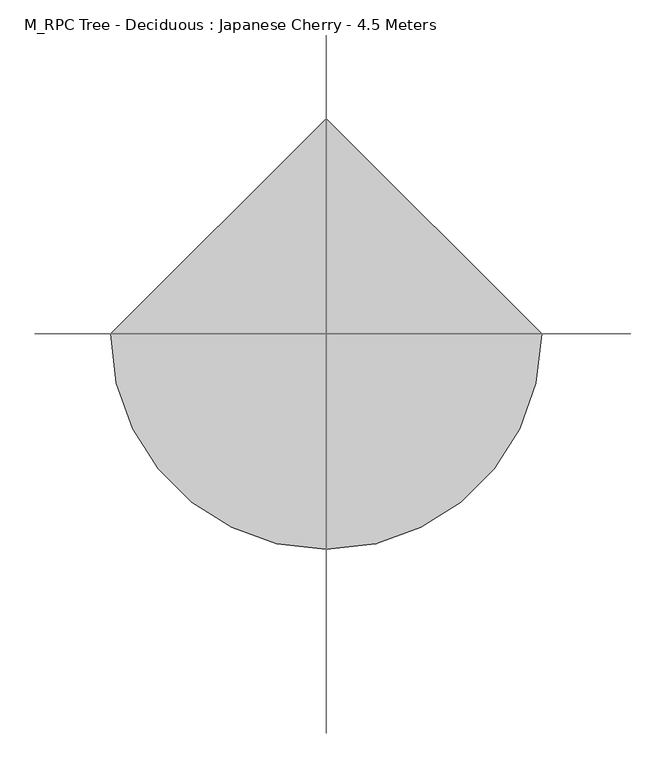
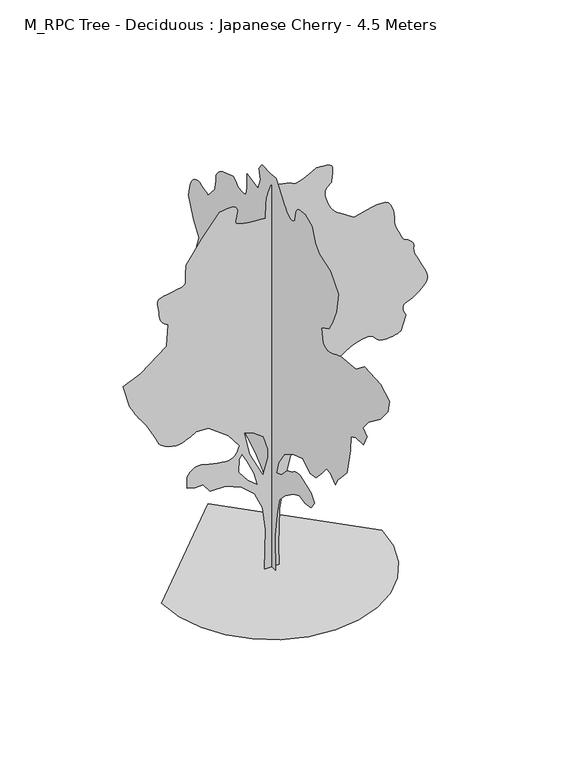
"""IFC4 building model written with IfcOpenShell, lengths in millimetres: geographic element geometry, M_RPC Tree - Deciduous : Japanese Cherry - 4.5 Meters."""

from ifc_helpers import new_model, si_unit, origin, place, context, project, spatial, triangles, source, transform, mapped, element, save


def m_rpc_tree_deciduous_japanese_cherry_4_5_meters_7aaeb41d(model_context):
    return source(origin(), model_context, "Body", "Tessellation", [
        triangles([(-0.0027587, 74.5725603, 0.00586), (-0.0027587, -72.0943095, 0.00586), (-0.0027587, -58.7610481, 393.3378007), (-0.0027587, -98.7608322, 653.338028), (-0.0027587, -145.4276149, 853.3381748), (-0.0027587, -252.0952047, 966.670792), (-0.0027587, -412.0928332, 1080.00588), (-0.0027587, -518.7604139, 1126.6709095), (-0.0027587, -625.428031, 1106.6708948), (-0.0027587, -738.7605755, 1126.6709095), (-0.0027587, -798.7606195, 1213.3385118), (-0.0027587, -738.7605755, 1293.3384979), (-0.0027587, -525.4279212, 1366.6710857), (-0.0027587, -506.885412, 1365.1761189), (-0.0027587, -488.5178922, 1363.2711479), (-0.0027587, -470.5003873, 1360.5486397), (-0.0027587, -453.0078504, 1356.6035316), (-0.0027587, -436.2153434, 1351.0261105), (-0.0027587, -420.2953485, 1343.4060814), (-0.0027587, -405.4278331, 1333.3385273), (-0.0027587, -390.5578105, 1322.4935497), (-0.0027587, -374.6402864, 1312.6960373), (-0.0027587, -357.8477795, 1303.7760876), (-0.0027587, -340.3552789, 1295.553479), (-0.0027587, -322.337774, 1287.8585999), (-0.0027587, -303.9702541, 1280.5110832), (-0.0027587, -285.4277268, 1273.3385559), (-0.0027587, -185.427399, 1166.6709389), (-0.0027587, -85.4275708, 1126.6709095), (-0.0027587, -125.4276002, 1266.671085), (-0.0027587, -238.7606988, 1433.3386734), (-0.0027587, -398.7603258, 1533.3386742), (-0.0027587, -585.4279653, 1593.3387909), (-0.0027587, -718.7605608, 1506.6712612), (-0.0027587, -825.4281778, 1520.0062031), (-0.0027587, -938.7607224, 1640.0038204), (-0.0027587, -1025.4283247, 1746.6714375), (-0.0027587, -1105.4259127, 1740.0039665), (-0.0027587, -1192.0934423, 1660.0063786), (-0.0027587, -1245.4260155, 1753.3389084), (-0.0027587, -1305.4259869, 1820.0040253), (-0.0027587, -1412.0936039, 1933.3391132), (-0.0027587, -1478.7587208, 2233.3392609), (-0.0027587, -1485.4261917, 2393.3393784), (-0.0027587, -1578.7613377, 2433.336937), (-0.0027587, -1725.426368, 2446.6718788), (-0.0027587, -1785.4264847, 2573.3269386), (-0.0027587, -1712.0938969, 2633.3270554), (-0.0027587, -1812.0938976, 2753.3272888), (-0.0027587, -2038.759132, 2926.6774635), (-0.0027587, -2185.4267784, 3100.0026398), (-0.0027587, -2212.0917206, 3240.0025246), (-0.0027587, -2045.4266029, 3333.3276421), (-0.0027587, -1738.758839, 3346.6776993), (-0.0027587, -1585.4263378, 3226.6774658), (-0.0027587, -1292.0935158, 3193.3274666), (-0.0027587, -1252.2485641, 3177.7025482), (-0.0027587, -1213.3385118, 3162.6025978), (-0.0027587, -1176.2909185, 3148.5525833), (-0.0027587, -1142.0459158, 3136.0774727), (-0.0027587, -1111.5309179, 3125.7025246), (-0.0027587, -1085.6808969, 3117.9524162), (-0.0027587, -1065.4258833, 3113.3274078), (-0.0027587, -1047.2933418, 3113.0774231), (-0.0027587, -1028.108321, 3117.0274727), (-0.0027587, -1009.2758223, 3123.6526497), (-0.0027587, -992.1908186, 3131.4524643), (-0.0027587, -978.255768, 3138.9025909), (-0.0027587, -968.8682596, 3144.4775414), (-0.0027587, -965.4258099, 3146.6774071), (-0.0027587, -932.0932514, 3306.6778152), (-0.0027587, -1072.0933542, 3380.0027), (-0.0027587, -1138.7609419, 3486.6778748), (-0.0027587, -1212.093457, 3660.003051), (-0.0027587, -1252.0934864, 3880.0029945), (-0.0027587, -1098.7609125, 4053.3281708), (-0.0027587, -898.760693, 4126.6783447), (-0.0027587, -818.7606342, 4200.0035202), (-0.0027587, -758.7605902, 4360.0036377), (-0.0027587, -618.7604874, 4413.3285805), (-0.0027587, -595.9604982, 4413.2285866), (-0.0027587, -573.5129585, 4412.5536278), (-0.0027587, -551.7629416, 4410.70345), (-0.0027587, -531.0629333, 4407.1286682), (-0.0027587, -511.7629123, 4401.17845), (-0.0027587, -494.2128934, 4392.3534073), (-0.0027587, -478.7603846, 4380.0035797), (-0.0027587, -466.2228868, 4364.5536507), (-0.0027587, -456.8353784, 4347.0035591), (-0.0027587, -450.0728551, 4327.7035744), (-0.0027587, -445.4078419, 4307.0033844), (-0.0027587, -442.3178415, 4285.2535492), (-0.0027587, -440.2753427, 4262.803466), (-0.0027587, -438.7603552, 4240.0034042), (-0.0027587, -427.2553525, 4227.3033073), (-0.0027587, -415.2803204, 4215.6034401), (-0.0027587, -402.3753304, 4205.9034508), (-0.0027587, -388.070317, 4199.1532814), (-0.0027587, -371.9003011, 4196.3784508), (-0.0027587, -353.3952896, 4198.553318), (-0.0027587, -332.0927745, 4206.6784035), (-0.0027587, -310.9852693, 4218.4782646), (-0.0027587, -293.0277353, 4231.0033722), (-0.0027587, -277.6927156, 4244.1034447), (-0.0027587, -264.4552061, 4257.6784882), (-0.0027587, -252.7927094, 4271.5785118), (-0.0027587, -242.1814384, 4285.7285202), (-0.0027587, -232.0939364, 4300.003521), (-0.0027587, -138.7608616, 4426.6786377), (-0.0027587, -78.7608175, 4500.0035225), (-0.0027587, 21.2393172, 4493.3286392), (-0.0027587, 181.2391554, 4500.0035225), (-0.0027587, 241.2389451, 4420.0034637), (-0.0027587, 214.5724224, 4306.6784042), (-0.0027587, 261.2402133, 4180.0032875), (-0.0027587, 467.9053785, 4220.0034622), (-0.0027587, 467.9053785, 4073.3284035), (-0.0027587, 469.4403866, 4050.6283356), (-0.0027587, 471.6178699, 4028.7032204), (-0.0027587, 475.0778695, 4008.4282951), (-0.0027587, 480.4628969, 3990.6282188), (-0.0027587, 488.4103769, 3976.0532364), (-0.0027587, 499.5679081, 3965.5782944), (-0.0027587, 514.5729152, 3960.0030533), (-0.0027587, 531.7154371, 3957.9281799), (-0.0027587, 548.8579591, 3957.2532211), (-0.0027587, 566.0004447, 3957.7281921), (-0.0027587, 583.1429667, 3959.1531052), (-0.0027587, 600.2854886, 3961.2782661), (-0.0027587, 617.4304813, 3963.853109), (-0.0027587, 634.5730396, 3966.6782272), (-0.0027587, 650.2955538, 3982.2281502), (-0.0027587, 666.0780207, 3996.928125), (-0.0027587, 681.9780676, 4009.8782066), (-0.0027587, 698.0505604, 4020.2031578), (-0.0027587, 714.3580679, 4027.0283226), (-0.0027587, 730.9580721, 4029.4781731), (-0.0027587, 747.9055841, 4026.678344), (-0.0027587, 927.9057163, 3966.6782272), (-0.0027587, 953.4457998, 3949.4781143), (-0.0027587, 977.9358021, 3931.9283134), (-0.0027587, 1000.3257872, 3913.6782646), (-0.0027587, 1019.5682899, 3894.3782799), (-0.0027587, 1034.6108311, 3873.6780899), (-0.0027587, 1044.4058727, 3851.2280067), (-0.0027587, 1047.9058771, 3826.6780518), (-0.0027587, 1048.6833733, 3801.5281334), (-0.0027587, 1050.8608566, 3777.4531494), (-0.0027587, 1054.2033852, 3754.253112), (-0.0027587, 1058.4783422, 3731.7530319), (-0.0027587, 1063.4533293, 3709.7529213), (-0.0027587, 1068.895875, 3688.1280785), (-0.0027587, 1074.570892, 3666.6779343), (-0.0027587, 1201.238451, 3526.6777588), (-0.0027587, 1239.7609543, 3543.5528915), (-0.0027587, 1277.9935043, 3558.9278252), (-0.0027587, 1315.641061, 3571.2779434), (-0.0027587, 1352.4135258, 3579.077758), (-0.0027587, 1388.0210907, 3580.8029434), (-0.0027587, 1422.1711864, 3574.9530098), (-0.0027587, 1454.5712437, 3560.0027596), (-0.0027587, 1482.6961258, 3536.9027161), (-0.0027587, 1504.8736965, 3508.1777252), (-0.0027587, 1522.093721, 3474.8027275), (-0.0027587, 1535.3487259, 3437.7026665), (-0.0027587, 1545.6312378, 3397.8027763), (-0.0027587, 1553.9313126, 3356.02771), (-0.0027587, 1561.2387154, 3313.3277), (-0.0027587, 1474.5711857, 3086.677581), (-0.0027587, 1367.9060394, 2940.0022316), (-0.0027587, 1454.5712437, 2700.0020554), (-0.0027587, 1374.5710396, 2573.3269386), (-0.0027587, 1341.9185268, 2561.8270592), (-0.0027587, 1310.4910847, 2549.851918), (-0.0027587, 1281.5110222, 2536.952124), (-0.0027587, 1256.2035553, 2522.6521248), (-0.0027587, 1235.7959347, 2506.4769493), (-0.0027587, 1221.5110508, 2487.9745903), (-0.0027587, 1214.5709948, 2466.6721115), (-0.0027587, 1212.2984591, 2444.0095413), (-0.0027587, 1211.0734612, 2421.694479), (-0.0027587, 1210.7234825, 2399.6744568), (-0.0027587, 1211.0734612, 2377.8869785), (-0.0027587, 1211.9484804, 2356.2718735), (-0.0027587, 1213.1734783, 2334.7768192), (-0.0027587, 1214.5709948, 2313.3368488), (-0.0027587, 1187.9059799, 2206.6718479), (-0.0027587, 1001.2383041, 2226.6717899), (-0.0027587, 985.728277, 2195.3792233), (-0.0027587, 971.4433205, 2164.9017231), (-0.0027587, 959.6057436, 2136.0592976), (-0.0027587, 951.4432331, 2109.6642517), (-0.0027587, 948.1782434, 2086.536739), (-0.0027587, 951.0357725, 2067.486739), (-0.0027587, 961.2382748, 2053.3392014), (-0.0027587, 977.7782536, 2041.5992203), (-0.0027587, 998.0507807, 2029.6266953), (-0.0027587, 1020.8883402, 2018.0041489), (-0.0027587, 1045.1258142, 2007.3141037), (-0.0027587, 1069.5958323, 1998.1390823), (-0.0027587, 1093.133349, 1991.0640781), (-0.0027587, 1114.5709213, 1986.6716137), (-0.0027587, 1133.9884134, 1982.8416149), (-0.0027587, 1152.3558969, 1977.2640484), (-0.0027587, 1169.8484339, 1970.229158), (-0.0027587, 1186.6409409, 1962.0266064), (-0.0027587, 1202.9109507, 1952.9491081), (-0.0027587, 1218.828511, 1943.2890873), (-0.0027587, 1234.5710094, 1933.3391132), (-0.0027587, 1387.9061268, 2013.339172), (-0.0027587, 1431.9861397, 2024.5916828), (-0.0027587, 1474.8436981, 2034.7965832), (-0.0027587, 1515.2512608, 2042.9016117), (-0.0027587, 1551.9862278, 2047.8566872), (-0.0027587, 1583.8238194, 2048.6141991), (-0.0027587, 1609.5388195, 2044.1266823), (-0.0027587, 1627.9038322, 2033.339114), (-0.0027587, 1640.0538174, 2017.6916679), (-0.0027587, 1648.351276, 1999.5965515), (-0.0027587, 1653.4438431, 1979.4615887), (-0.0027587, 1655.9713051, 1957.6915512), (-0.0027587, 1656.5738846, 1934.6990593), (-0.0027587, 1655.8938389, 1910.8890301), (-0.0027587, 1654.5713905, 1886.6714676), (-0.0027587, 1631.6563648, 1862.5890713), (-0.0027587, 1608.3913605, 1839.7339256), (-0.0027587, 1584.4262535, 1819.3239796), (-0.0027587, 1559.4112106, 1802.5889545), (-0.0027587, 1532.9962532, 1790.7539211), (-0.0027587, 1504.833728, 1785.0390083), (-0.0027587, 1474.5711857, 1786.6714668), (-0.0027587, 1442.5211071, 1793.7065025), (-0.0027587, 1410.0036152, 1802.1439236), (-0.0027587, 1378.1860806, 1810.1114605), (-0.0027587, 1348.2360191, 1815.7489071), (-0.0027587, 1321.3160053, 1817.1864647), (-0.0027587, 1298.5960258, 1812.5614563), (-0.0027587, 1281.2385098, 1800.0039379), (-0.0027587, 1268.1185257, 1783.8339947), (-0.0027587, 1257.0985588, 1769.4114738), (-0.0027587, 1247.8260143, 1756.448893), (-0.0027587, 1239.9560005, 1744.6513573), (-0.0027587, 1233.1334518, 1733.7264427), (-0.0027587, 1227.0110058, 1723.3863762), (-0.0027587, 1221.2385384, 1713.338879), (-0.0027587, 1243.9585178, 1710.3264175), (-0.0027587, 1265.8635761, 1706.3813095), (-0.0027587, 1286.1360306, 1700.5688736), (-0.0027587, 1303.9584892, 1691.958934), (-0.0027587, 1318.5160309, 1679.6163734), (-0.0027587, 1328.993589, 1662.608836), (-0.0027587, 1334.5710102, 1640.0038204), (-0.0027587, 1336.8460167, 1613.5138676), (-0.0027587, 1338.0710873, 1585.6212387), (-0.0027587, 1338.4210659, 1556.56371), (-0.0027587, 1338.0710873, 1526.5736801), (-0.0027587, 1337.1961407, 1495.8836929), (-0.0027587, 1335.9710701, 1464.7286179), (-0.0027587, 1334.5710102, 1433.3386734), (-0.0027587, 1300.3260075, 1407.8185741), (-0.0027587, 1266.3110779, 1383.4636654), (-0.0027587, 1232.7635616, 1361.4436432), (-0.0027587, 1199.9160027, 1342.9210819), (-0.0027587, 1168.0034157, 1329.0636429), (-0.0027587, 1137.2534031, 1321.0360806), (-0.0027587, 1107.9059212, 1320.0060562), (-0.0027587, 1078.5558958, 1323.638538), (-0.0027587, 1047.808354, 1328.6735504), (-0.0027587, 1015.8932962, 1334.873608), (-0.0027587, 983.0458099, 1342.0060215), (-0.0027587, 949.4982937, 1349.8411537), (-0.0027587, 915.4857622, 1358.1386124), (-0.0027587, 881.238216, 1366.6710857), (-0.0027587, 681.2380692, 1320.0060562), (-0.0027587, 447.9053638, 1200.0059681), (-0.0027587, 314.5727683, 1126.6709095), (-0.0027587, 161.2391225, 1000.0058212), (-0.0027587, 67.905807, 806.6731453), (-0.0027587, 41.2392842, 533.3379398), (-0.0027587, 67.905807, 260.0052052), (78.9470616, 0.0002511, 0.0), (-81.0528197, 0.0002511, 0.0), (-67.7195538, 0.0002197, 453.3328669), (-101.05258, 0.0001988, 713.3330578), (-187.7194103, 0.0001884, 899.9982628), (-327.7202579, 0.0001884, 1026.6658218), (-501.0529192, 0.0001779, 1099.9984097), (-667.7180368, 0.0001779, 1099.9984097), (-747.720639, 0.0001779, 1199.9984831), (-834.3856979, 0.0001779, 1199.9984831), (-921.0532276, 0.0001779, 1219.9984978), (-921.0532276, 0.0001674, 1346.6660568), (-903.7932346, 0.0001674, 1369.3085701), (-885.8332117, 0.0001674, 1390.6686035), (-866.4756723, 0.000157, 1409.4636772), (-845.0181885, 0.000157, 1424.411166), (-820.7606575, 0.000157, 1434.2261192), (-793.0056656, 0.000157, 1437.6286732), (-761.0531101, 0.000157, 1433.3335865), (-723.1130568, 0.000157, 1423.7311203), (-679.5755253, 0.000157, 1412.8461742), (-633.0054754, 0.0001674, 1401.8461189), (-585.970483, 0.0001674, 1391.8936741), (-541.032928, 0.0001674, 1384.1586811), (-500.7604225, 0.0001674, 1379.803569), (-467.71789, 0.0001674, 1379.9986153), (-441.4803563, 0.0001674, 1385.9661289), (-419.4403499, 0.0001674, 1397.5311207), (-400.8978407, 0.000157, 1413.7610893), (-385.1527988, 0.000157, 1433.7212082), (-371.5103176, 0.000157, 1456.4811562), (-359.2652802, 0.000157, 1481.1062519), (-347.7202726, 0.000157, 1506.6661743), (-467.71789, 0.0001465, 1666.6662918), (-687.7180515, 0.000136, 1826.6664093), (-821.0531542, 0.000136, 1833.3314095), (-842.5681927, 0.000136, 1820.5039948), (-864.6081991, 0.000136, 1807.851424), (-887.7006849, 0.000136, 1795.5489773), (-912.3632057, 0.000136, 1783.7688824), (-939.1282871, 0.000136, 1772.6913609), (-968.5158102, 0.000136, 1762.4864605), (-1001.0532864, 0.0001465, 1753.3313507), (-1038.4858126, 0.0001465, 1750.1639568), (-1080.1183731, 0.0001465, 1756.5589153), (-1122.8009422, 0.000136, 1770.6488983), (-1163.385965, 0.000136, 1790.5713741), (-1198.7209448, 0.000136, 1814.4590149), (-1225.6584721, 0.000136, 1840.4465275), (-1241.0509918, 0.000136, 1866.6664387), (-1254.4834568, 0.000136, 1899.3565945), (-1275.8434902, 0.0001256, 1942.8940533), (-1302.4510231, 0.0001256, 1992.6141289), (-1331.6261318, 0.0001256, 2043.8466122), (-1360.6836605, 0.0001256, 2091.9317585), (-1386.9410694, 0.0001151, 2132.204155), (-1407.7185802, 0.0001151, 2159.9992607), (-1425.2510857, 0.0001151, 2182.1367176), (-1443.4812229, 0.0001151, 2208.1242302), (-1462.2962082, 0.0001151, 2237.3167797), (-1481.576136, 0.0001151, 2269.0742889), (-1501.2061878, 0.0001046, 2302.7592968), (-1521.0712543, 0.0001046, 2337.7244591), (-1541.0512848, 0.0001046, 2373.3318787), (-1614.3863434, 9.42e-05, 2626.6771706), (-1421.0511967, 8.37e-05, 2706.6772293), (-1141.0533892, 7.32e-05, 2926.6774635), (-1127.7183746, 5.23e-05, 3166.6526413), (-1147.5834412, 5.23e-05, 3181.0776329), (-1166.6309704, 5.23e-05, 3196.1775833), (-1184.0459684, 5.23e-05, 3212.677739), (-1199.0109707, 5.23e-05, 3231.2774757), (-1210.7109833, 5.23e-05, 3252.677623), (-1218.3310123, 5.23e-05, 3277.5775566), (-1221.0535206, 5.23e-05, 3306.6525261), (-1223.4635479, 4.19e-05, 3339.402562), (-1228.9034775, 4.19e-05, 3373.552803), (-1234.6960018, 4.19e-05, 3407.2527809), (-1238.155965, 4.19e-05, 3438.6029022), (-1236.6009727, 4.19e-05, 3465.7526985), (-1227.3484852, 4.19e-05, 3486.8278656), (-1207.7185061, 4.19e-05, 3500.0029335), (-1173.335939, 4.19e-05, 3508.2777191), (-1126.1258846, 3.14e-05, 3516.4528015), (-1072.8508661, 3.14e-05, 3525.1778503), (-1020.2758049, 3.14e-05, 3535.2278183), (-975.1632969, 3.14e-05, 3547.2279579), (-944.2782635, 3.14e-05, 3561.9279327), (-934.3857714, 3.14e-05, 3580.0029922), (-936.4657316, 3.14e-05, 3601.7528275), (-937.1457773, 3.14e-05, 3626.6530518), (-936.6582344, 3.14e-05, 3654.1778252), (-935.2407337, 3.14e-05, 3683.7780533), (-933.1232758, 2.09e-05, 3714.9778931), (-930.5382591, 2.09e-05, 3747.2279594), (-927.7182278, 2.09e-05, 3780.0029938), (-761.0531101, 1.05e-05, 4020.00317), (-567.7204705, -1.05e-05, 4260.0033463), (-526.5729095, -1.05e-05, 4266.8535095), (-487.1179049, -1.05e-05, 4272.0284843), (-451.042854, -1.05e-05, 4273.8283745), (-420.0428567, -1.05e-05, 4270.5285759), (-395.80531, -1.05e-05, 4260.4783173), (-380.0228067, -1.05e-05, 4241.9782837), (-374.3852875, 0.0, 4213.3282883), (-377.165314, 0.0, 4181.0535141), (-383.5603088, 0.0, 4152.6032158), (-390.6553336, 0.0, 4127.8032761), (-395.5328339, 0.0, 4106.3534225), (-395.2803057, 0.0, 4088.0533768), (-386.9803036, 0.0, 4072.6781525), (-367.7202873, 0.0, 4060.0033447), (-338.5077899, 0.0, 4049.7283905), (-302.995241, 0.0, 4041.5783066), (-262.2377179, 1.05e-05, 4035.1531174), (-217.282177, 1.05e-05, 4030.1531319), (-169.1771373, 1.05e-05, 4026.1783745), (-118.9730978, 1.05e-05, 4022.9032837), (-67.7195538, 1.05e-05, 4020.00317), (-61.0525507, 0.0, 4200.0035202), (-59.4975493, -1.05e-05, 4225.5284157), (-55.1437952, -1.05e-05, 4250.678334), (-48.4577889, -1.05e-05, 4275.5535599), (-39.9057809, -1.05e-05, 4300.2035088), (-29.954274, -1.05e-05, 4324.6784683), (-19.070066, -1.05e-05, 4349.0284355), (-7.719256, -1.05e-05, 4373.3284058), (37.7812808, -1.05e-05, 4364.72864), (81.9990646, -1.05e-05, 4356.0285896), (123.6511007, -1.05e-05, 4347.103553), (161.4548797, -1.05e-05, 4337.8035393), (194.127413, -1.05e-05, 4328.053553), (220.3859302, -1.05e-05, 4317.7036034), (238.9474425, -1.05e-05, 4306.6534058), (263.1077047, -1.05e-05, 4303.4286026), (302.4252358, -1.05e-05, 4313.503569), (350.0252918, -1.05e-05, 4332.2035904), (399.0253169, -1.05e-05, 4354.8786598), (442.5428641, -1.05e-05, 4376.8284828), (473.6978665, -2.09e-05, 4393.4286324), (485.6129096, -2.09e-05, 4400.0035217), (495.2154121, -2.09e-05, 4400.2035095), (519.9779268, -2.09e-05, 4399.9285263), (553.8354532, -2.09e-05, 4397.9036499), (590.7254617, -2.09e-05, 4392.8536674), (624.5830244, -1.05e-05, 4383.4786583), (649.3455391, -1.05e-05, 4368.5034096), (658.9480053, -1.05e-05, 4346.6535805), (658.5580582, -1.05e-05, 4321.3283821), (657.4705519, -1.05e-05, 4296.7034317), (655.7980522, -1.05e-05, 4272.6784447), (653.6605373, -1.05e-05, 4249.1034302), (651.1730438, -1.05e-05, 4225.8783943), (648.4505356, 0.0, 4202.8783447), (645.6129908, 0.0, 4180.0032875), (628.6255102, 0.0, 4167.0034996), (612.5730017, 0.0, 4153.2784653), (598.3829885, 0.0, 4138.0032349), (586.992986, 0.0, 4120.4784325), (579.3354592, 0.0, 4099.9282333), (576.342982, 0.0, 4075.5782661), (578.9479829, 0.0, 4046.6532875), (586.2154899, 1.05e-05, 4014.6032089), (596.2829713, 1.05e-05, 3981.953167), (608.6854846, 1.05e-05, 3949.7530975), (622.9504932, 1.05e-05, 3919.0782257), (638.6155254, 1.05e-05, 3890.9781967), (655.2155296, 1.05e-05, 3866.4782387), (672.280549, 2.09e-05, 3846.6529953), (692.3380457, 2.09e-05, 3828.553228), (717.6455853, 2.09e-05, 3808.6779877), (747.3231342, 2.09e-05, 3787.3531265), (780.5031584, 2.09e-05, 3764.8780449), (816.3031534, 2.09e-05, 3741.5030182), (853.853187, 2.09e-05, 3717.5780251), (892.2807106, 2.09e-05, 3693.3280518), (959.140801, 2.09e-05, 3711.6280975), (1024.3108057, 2.09e-05, 3728.2279564), (1086.098386, 2.09e-05, 3741.4280228), (1142.8159269, 2.09e-05, 3749.5781067), (1192.7659304, 2.09e-05, 3750.9530228), (1234.2634701, 2.09e-05, 3743.8781639), (1265.6135914, 2.09e-05, 3726.6530525), (1288.19855, 2.09e-05, 3698.6530174), (1305.0685959, 3.14e-05, 3662.6028923), (1317.0411209, 3.14e-05, 3621.8780525), (1324.9335171, 3.14e-05, 3579.8779999), (1329.5585255, 3.14e-05, 3539.9778191), (1331.7360088, 4.19e-05, 3505.5528854), (1332.2810337, 4.19e-05, 3480.0027008), (1337.451067, 4.19e-05, 3452.7529106), (1350.7835381, 4.19e-05, 3414.6526199), (1369.0136753, 4.19e-05, 3371.2026558), (1388.8785965, 5.23e-05, 3327.8526855), (1407.1112045, 5.23e-05, 3290.1026642), (1420.4436756, 5.23e-05, 3263.4275482), (1425.6137089, 5.23e-05, 3253.3275833), (1432.59119, 5.23e-05, 3250.5527527), (1450.4136486, 5.23e-05, 3242.5276611), (1474.4187241, 5.23e-05, 3229.7275703), (1499.938678, 5.23e-05, 3212.6024529), (1522.3086788, 5.23e-05, 3191.6275703), (1536.8662205, 5.23e-05, 3167.2776031), (1538.9461807, 6.28e-05, 3140.0025238), (1536.3412525, 6.28e-05, 3112.1024826), (1539.3362732, 6.28e-05, 3085.0273911), (1546.9938, 6.28e-05, 3057.9525902), (1558.3838024, 6.28e-05, 3030.0775475), (1572.5713085, 6.28e-05, 3000.5523148), (1588.6262878, 7.32e-05, 2968.5775223), (1605.6137684, 7.32e-05, 2933.3273483), (1625.0112762, 7.32e-05, 2895.102356), (1646.5088013, 7.32e-05, 2855.2271736), (1666.4888317, 7.32e-05, 2814.5523308), (1681.3363266, 8.37e-05, 2773.8771973), (1687.4413319, 8.37e-05, 2734.0023056), (1681.1813942, 8.37e-05, 2695.7773132), (1658.9462688, 8.37e-05, 2660.0021713), (1628.9963528, 9.42e-05, 2628.8270393), (1601.3762363, 9.42e-05, 2603.2521469), (1575.1563251, 9.42e-05, 2582.3269707), (1549.4036819, 9.42e-05, 2565.1521469), (1523.1837708, 9.42e-05, 2550.7771523), (1495.5662704, 9.42e-05, 2538.2520447), (1465.6137383, 9.42e-05, 2526.6771698), (1440.211219, 9.42e-05, 2513.3021141), (1425.6512066, 9.42e-05, 2496.4220398), (1420.1311947, 9.42e-05, 2476.6369102), (1421.8435902, 0.0001046, 2454.5170395), (1428.976149, 0.0001046, 2430.6494556), (1439.7236034, 0.0001046, 2405.616972), (1452.2811218, 0.0001046, 2379.9993496), (1398.9461506, 0.0001151, 2213.3317612), (1380.1910454, 0.0001151, 2204.8392563), (1360.3261242, 0.0001151, 2196.8118393), (1338.2460766, 0.0001151, 2189.7167782), (1312.8435574, 0.0001151, 2184.021777), (1283.0086052, 0.0001151, 2180.194249), (1247.6334389, 0.0001151, 2178.6968113), (1205.6134747, 0.0001151, 2179.9992027), (1167.8684675, 0.0001151, 2188.6467854), (1142.0184465, 0.0001151, 2205.9268353), (1121.9983749, 0.0001151, 2227.4043034), (1101.7459047, 0.0001151, 2248.6467567), (1075.1958538, 0.0001151, 2265.2268494), (1036.2833307, 0.0001151, 2272.7093868), (978.9457695, 0.0001151, 2266.6642616), (912.6507608, 0.0001151, 2247.8318356), (851.8331795, 0.0001151, 2221.3017689), (797.8981722, 0.0001151, 2189.1717533), (752.2406393, 0.0001151, 2153.5467476), (716.2655823, 0.0001151, 2116.5192112), (691.365576, 0.0001256, 2080.1942482), (678.94802, 0.0001256, 2046.6666435), (678.6755802, 0.0001256, 2016.7915775), (688.1980368, 0.0001256, 1989.7166313), (705.8855473, 0.0001256, 1964.9741009), (730.1031097, 0.0001256, 1942.0990437), (759.2181204, 0.000136, 1920.6215755), (791.6006641, 0.000136, 1900.0764633), (825.6131956, 0.000136, 1879.9990551), (845.4582052, 0.000136, 1867.0540604), (864.3707136, 0.000136, 1853.5839523), (881.4156761, 0.000136, 1839.0665245), (895.6632076, 0.000136, 1822.9739021), (906.1782635, 0.000136, 1804.7814079), (912.0282698, 0.000136, 1783.9639286), (912.2807253, 0.000136, 1759.998967), (909.6182425, 0.0001465, 1730.7863605), (907.3057383, 0.0001465, 1695.2763187), (905.28326, 0.0001465, 1654.5187775), (903.4957237, 0.0001465, 1609.5613472), (901.880706, 0.000157, 1561.4562893), (900.3857391, 0.000157, 1511.253685), (898.9457108, 0.000157, 1459.998674), (864.6231691, 0.000157, 1434.5760979), (830.0656855, 0.000157, 1410.9037056), (795.0406431, 0.0001674, 1390.7286289), (759.3156435, 0.0001674, 1375.8010517), (722.6606134, 0.0001674, 1367.8711578), (684.835524, 0.0001674, 1368.686079), (645.6129908, 0.0001674, 1379.9986153), (606.1979911, 0.0001674, 1395.0036587), (567.8304565, 0.0001674, 1406.1611172), (530.3354342, 0.000157, 1414.1112133), (493.5429125, 0.000157, 1419.4935883), (457.2753588, 0.000157, 1422.9536968), (421.3578564, 0.000157, 1425.1311802), (385.6127998, 0.000157, 1426.6661156), (272.280219, 0.0001674, 1353.3335278), (198.9474132, 0.0001779, 1186.6659393), (125.6138534, 0.0001884, 906.6657337), (85.6140693, 0.0002093, 633.332999), (72.2805581, 0.0002302, 233.3331958), (-94.386072, 8.37e-05, 1079.998395), (-41.0527812, 7.32e-05, 1266.6659981), (-41.0527812, 6.28e-05, 1359.9985279), (-87.7190734, 5.23e-05, 1519.9987907), (-207.7189163, 5.23e-05, 1606.6663204), (-301.052736, 5.23e-05, 1639.9988789), (-241.0526919, 6.28e-05, 1373.3336151), (-154.3856164, 6.28e-05, 993.3333361), (-194.385664, 6.28e-05, 1139.998439), (-267.7202139, 5.23e-05, 1299.9985565), (-321.0527507, 4.19e-05, 1399.9987026), (-354.3852728, 4.19e-05, 1353.3335278), (-361.0527801, 5.23e-05, 1206.665954), (-261.0527066, 6.28e-05, 1079.998395), (-1193.8159389, 0.0, 0.0045206), (-1162.2559467, -273.5427146, 0.0045206), (-1072.3708809, -524.7504189, 0.0045206), (-931.360738, -746.420573, 0.0045206), (-746.420573, -931.360738, 0.0045206), (-524.7504189, -1072.3708809, 0.0045206), (-273.5427146, -1162.2559467, 0.0045206), (5.22e-05, -1193.8159389, 0.0045206), (273.5427146, -1162.2559467, 0.0045206), (524.7504189, -1072.3708809, 0.0045206), (746.420573, -931.360738, 0.0045206), (931.360738, -746.420573, 0.0045206), (1072.3708809, -524.7504189, 0.0045206), (1162.2559467, -273.5427146, 0.0045206), (1193.8159389, 0.0001046, 0.0045206), (-0.0001566, 1193.8159389, 0.0045206)], [[38, 39, 40], [115, 116, 117], [1, 2, 3], [280, 1, 3], [279, 280, 3], [279, 3, 4], [278, 279, 4], [278, 4, 5], [186, 187, 188], [277, 278, 5], [46, 47, 48], [45, 46, 48], [277, 5, 6], [185, 186, 188], [10, 11, 12], [9, 10, 12], [9, 12, 13], [8, 9, 13], [8, 13, 14], [8, 14, 15], [8, 15, 16], [8, 16, 17], [8, 17, 18], [8, 18, 19], [8, 19, 20], [8, 20, 21], [7, 8, 21], [7, 21, 22], [7, 22, 23], [7, 23, 24], [7, 24, 25], [7, 25, 26], [6, 7, 26], [6, 26, 27], [6, 27, 28], [277, 6, 28], [277, 28, 29], [51, 52, 53], [50, 51, 53], [50, 53, 54], [50, 54, 55], [49, 50, 55], [49, 55, 56], [48, 49, 56], [48, 56, 57], [45, 48, 57], [44, 45, 57], [44, 57, 58], [44, 58, 59], [44, 59, 60], [44, 60, 61], [44, 61, 62], [44, 62, 63], [276, 277, 29], [276, 29, 30], [184, 185, 188], [183, 184, 188], [44, 63, 64], [115, 117, 118], [111, 112, 113], [111, 113, 114], [182, 183, 188], [109, 110, 111], [109, 111, 114], [108, 109, 114], [108, 114, 115], [107, 108, 115], [106, 107, 115], [105, 106, 115], [104, 105, 115], [115, 118, 119], [170, 171, 172], [170, 172, 173], [170, 173, 174], [170, 174, 175], [74, 75, 76], [74, 76, 77], [73, 74, 77], [72, 73, 77], [71, 72, 77], [258, 259, 260], [181, 182, 188], [78, 79, 80], [170, 175, 176], [103, 104, 115], [78, 80, 81], [44, 64, 65], [275, 276, 30], [275, 30, 31], [274, 275, 31], [78, 81, 82], [78, 82, 83], [78, 83, 84], [78, 84, 85], [78, 85, 86], [78, 86, 87], [78, 87, 88], [78, 88, 89], [78, 89, 90], [78, 90, 91], [78, 91, 92], [78, 92, 93], [78, 93, 94], [78, 94, 95], [78, 95, 96], [71, 77, 78], [71, 78, 96], [71, 96, 97], [71, 97, 98], [71, 98, 99], [71, 99, 100], [115, 119, 120], [180, 181, 188], [38, 40, 41], [223, 224, 225], [33, 34, 35], [33, 35, 36], [33, 36, 37], [102, 103, 115], [179, 180, 188], [44, 65, 66], [170, 176, 177], [71, 100, 101], [43, 44, 66], [42, 43, 66], [41, 42, 66], [38, 41, 66], [37, 38, 66], [33, 37, 66], [33, 66, 67], [33, 67, 68], [33, 68, 69], [33, 69, 70], [32, 33, 70], [31, 32, 70], [274, 31, 70], [273, 274, 70], [273, 70, 71], [273, 71, 101], [273, 101, 102], [273, 102, 115], [273, 115, 120], [273, 120, 121], [273, 121, 122], [273, 122, 123], [273, 123, 124], [273, 124, 125], [273, 125, 126], [273, 126, 127], [273, 127, 128], [273, 128, 129], [273, 129, 130], [273, 130, 131], [272, 273, 131], [271, 272, 131], [270, 271, 131], [269, 270, 131], [268, 269, 131], [268, 131, 132], [268, 132, 133], [268, 133, 134], [167, 168, 169], [257, 258, 260], [257, 260, 261], [256, 257, 261], [256, 261, 262], [255, 256, 262], [255, 262, 263], [254, 255, 263], [254, 263, 264], [254, 264, 265], [254, 265, 266], [254, 266, 267], [254, 267, 268], [253, 254, 268], [252, 253, 268], [251, 252, 268], [250, 251, 268], [249, 250, 268], [248, 249, 268], [247, 248, 268], [246, 247, 268], [245, 246, 268], [166, 167, 169], [165, 166, 169], [164, 165, 169], [163, 164, 169], [162, 163, 169], [161, 162, 169], [160, 161, 169], [159, 160, 169], [158, 159, 169], [157, 158, 169], [156, 157, 169], [155, 156, 169], [154, 155, 169], [154, 169, 170], [154, 170, 177], [153, 154, 177], [153, 177, 178], [153, 178, 179], [153, 179, 188], [222, 223, 225], [222, 225, 226], [221, 222, 226], [220, 221, 226], [219, 220, 226], [218, 219, 226], [217, 218, 226], [216, 217, 226], [215, 216, 226], [214, 215, 226], [213, 214, 226], [212, 213, 226], [212, 226, 227], [212, 227, 228], [212, 228, 229], [212, 229, 230], [212, 230, 231], [211, 212, 231], [211, 231, 232], [211, 232, 233], [210, 211, 233], [209, 210, 233], [209, 233, 234], [209, 234, 235], [209, 235, 236], [209, 236, 237], [209, 237, 238], [209, 238, 239], [209, 239, 240], [208, 209, 240], [208, 240, 241], [207, 208, 241], [206, 207, 241], [206, 241, 242], [205, 206, 242], [204, 205, 242], [204, 242, 243], [203, 204, 243], [202, 203, 243], [202, 243, 244], [201, 202, 244], [201, 244, 245], [201, 245, 268], [200, 201, 268], [199, 200, 268], [198, 199, 268], [197, 198, 268], [196, 197, 268], [195, 196, 268], [194, 195, 268], [153, 188, 189], [153, 189, 190], [152, 153, 190], [152, 190, 191], [151, 152, 191], [136, 137, 138], [135, 136, 138], [135, 138, 139], [134, 135, 139], [134, 139, 140], [134, 140, 141], [134, 141, 142], [134, 142, 143], [134, 143, 144], [134, 144, 145], [134, 145, 146], [134, 146, 147], [134, 147, 148], [134, 148, 149], [134, 149, 150], [134, 150, 151], [134, 151, 191], [134, 191, 192], [134, 192, 193], [268, 134, 193], [194, 268, 193], [583, 580, 581], [574, 281, 575], [580, 583, 584], [573, 574, 575], [583, 581, 575], [580, 584, 585], [572, 573, 575], [582, 583, 575], [582, 575, 281], [571, 572, 575], [571, 575, 576], [281, 282, 283], [570, 571, 576], [570, 576, 577], [344, 345, 346], [290, 291, 292], [406, 407, 408], [570, 577, 578], [290, 292, 293], [289, 290, 293], [289, 293, 294], [289, 294, 295], [289, 295, 296], [289, 296, 297], [289, 297, 298], [289, 298, 299], [289, 299, 300], [289, 300, 301], [289, 301, 302], [289, 302, 303], [288, 289, 303], [287, 288, 303], [287, 303, 304], [287, 304, 305], [287, 305, 306], [286, 287, 306], [286, 306, 307], [286, 307, 308], [286, 308, 309], [569, 570, 578], [554, 555, 556], [405, 406, 408], [343, 344, 346], [512, 513, 514], [511, 512, 514], [511, 514, 515], [511, 515, 516], [511, 516, 517], [510, 511, 517], [510, 517, 518], [510, 518, 519], [510, 519, 520], [510, 520, 521], [510, 521, 522], [510, 522, 523], [510, 523, 524], [509, 510, 524], [509, 524, 525], [508, 509, 525], [434, 435, 436], [342, 343, 346], [507, 508, 525], [507, 525, 526], [405, 408, 409], [404, 405, 409], [403, 404, 409], [403, 409, 410], [402, 403, 410], [401, 402, 410], [400, 401, 410], [400, 410, 411], [399, 400, 411], [399, 411, 412], [399, 412, 413], [399, 413, 414], [399, 414, 415], [377, 378, 379], [341, 342, 346], [341, 346, 347], [340, 341, 347], [339, 340, 347], [338, 339, 347], [337, 338, 347], [336, 337, 347], [335, 336, 347], [334, 335, 347], [333, 334, 347], [377, 379, 380], [377, 380, 381], [377, 381, 382], [377, 382, 383], [377, 383, 384], [377, 384, 385], [377, 385, 386], [377, 386, 387], [377, 387, 388], [377, 388, 389], [377, 389, 390], [377, 390, 391], [376, 377, 391], [376, 391, 392], [375, 376, 392], [374, 375, 392], [373, 374, 392], [372, 373, 392], [372, 392, 393], [371, 372, 393], [370, 371, 393], [369, 370, 393], [369, 393, 394], [369, 394, 395], [369, 395, 396], [332, 333, 347], [369, 396, 397], [426, 427, 428], [426, 428, 429], [425, 426, 429], [425, 429, 430], [424, 425, 430], [424, 430, 431], [423, 424, 431], [423, 431, 432], [422, 423, 432], [422, 432, 433], [421, 422, 433], [420, 421, 433], [419, 420, 433], [418, 419, 433], [418, 433, 434], [418, 434, 436], [418, 436, 437], [418, 437, 438], [418, 438, 439], [417, 418, 439], [417, 439, 440], [416, 417, 440], [416, 440, 441], [415, 416, 441], [399, 415, 441], [399, 441, 442], [399, 442, 443], [399, 443, 444], [399, 444, 445], [399, 445, 446], [399, 446, 447], [399, 447, 448], [399, 448, 449], [369, 397, 398], [331, 332, 347], [368, 369, 398], [360, 361, 362], [359, 360, 362], [359, 362, 363], [358, 359, 363], [358, 363, 364], [357, 358, 364], [357, 364, 365], [356, 357, 365], [355, 356, 365], [355, 365, 366], [354, 355, 366], [353, 354, 366], [352, 353, 366], [351, 352, 366], [350, 351, 366], [349, 350, 366], [348, 349, 366], [348, 366, 367], [348, 367, 368], [348, 368, 398], [347, 348, 398], [347, 398, 399], [347, 399, 449], [347, 449, 450], [347, 450, 451], [347, 451, 452], [331, 347, 452], [331, 452, 453], [331, 453, 454], [331, 454, 455], [331, 455, 456], [330, 331, 456], [329, 330, 456], [328, 329, 456], [327, 328, 456], [326, 327, 456], [325, 326, 456], [324, 325, 456], [323, 324, 456], [322, 323, 456], [321, 322, 456], [320, 321, 456], [319, 320, 456], [318, 319, 456], [317, 318, 456], [316, 317, 456], [315, 316, 456], [314, 315, 456], [314, 456, 457], [314, 457, 458], [314, 458, 459], [314, 459, 460], [314, 460, 461], [314, 461, 462], [314, 462, 463], [314, 463, 464], [314, 464, 465], [314, 465, 466], [314, 466, 467], [314, 467, 468], [314, 468, 469], [314, 469, 470], [314, 470, 471], [314, 471, 472], [314, 472, 473], [314, 473, 474], [314, 474, 475], [314, 475, 476], [314, 476, 477], [314, 477, 478], [314, 478, 479], [314, 479, 480], [314, 480, 481], [314, 481, 482], [314, 482, 483], [314, 483, 484], [314, 484, 485], [314, 485, 486], [314, 486, 487], [314, 487, 488], [314, 488, 489], [314, 489, 490], [314, 490, 491], [314, 491, 492], [314, 492, 493], [314, 493, 494], [314, 494, 495], [314, 495, 496], [314, 496, 497], [314, 497, 498], [314, 498, 499], [314, 499, 500], [314, 500, 501], [314, 501, 502], [580, 585, 586], [554, 556, 557], [553, 554, 557], [553, 557, 558], [553, 558, 559], [553, 559, 560], [553, 560, 561], [553, 561, 562], [553, 562, 563], [552, 553, 563], [552, 563, 564], [551, 552, 564], [550, 551, 564], [550, 564, 565], [549, 550, 565], [549, 565, 566], [548, 549, 566], [547, 548, 566], [546, 547, 566], [545, 546, 566], [544, 545, 566], [543, 544, 566], [542, 543, 566], [541, 542, 566], [540, 541, 566], [539, 540, 566], [538, 539, 566], [538, 566, 567], [537, 538, 567], [537, 567, 568], [537, 568, 569], [537, 569, 578], [536, 537, 578], [535, 536, 578], [535, 578, 579], [534, 535, 579], [534, 579, 580], [533, 534, 580], [532, 533, 580], [507, 526, 527], [506, 507, 527], [531, 532, 580], [506, 527, 528], [530, 531, 580], [281, 283, 284], [582, 281, 284], [582, 284, 285], [582, 285, 286], [588, 582, 286], [587, 588, 286], [587, 286, 309], [586, 587, 309], [586, 309, 310], [586, 310, 311], [586, 311, 312], [586, 312, 313], [580, 586, 313], [580, 313, 314], [530, 580, 314], [529, 530, 314], [502, 503, 504], [502, 504, 505], [314, 502, 505], [529, 314, 505], [529, 505, 506], [529, 506, 528], [603, 604, 589], [602, 603, 589], [602, 589, 590], [601, 602, 590], [601, 590, 591], [601, 591, 592], [600, 601, 592], [599, 600, 592], [599, 592, 593], [599, 593, 594], [599, 594, 595], [599, 595, 596], [599, 596, 597], [599, 597, 598]], closed=False),
    ])


if __name__ == "__main__":
    model = new_model("IFC4")
    model_context = context("Model", 3, world=origin())
    ifc_project = project(units=[si_unit("LENGTHUNIT", "METRE", prefix="MILLI")], contexts=[model_context])
    site = spatial("IfcSite", under=ifc_project)
    building = spatial("IfcBuilding", under=site)
    placement = place(None, origin())
    m_rpc_tree_deciduous_japanese_cherry_4_5_meters_shape = m_rpc_tree_deciduous_japanese_cherry_4_5_meters_7aaeb41d(model_context)
    element("IfcGeographicElement", 1, ObjectType="M_RPC Tree - Deciduous : Japanese Cherry - 4.5 Meters", at=placement, inside=building, context=model_context, shape_type="MappedRepresentation", body=[
        mapped(m_rpc_tree_deciduous_japanese_cherry_4_5_meters_shape, transform((0.0, 0.0, 0.0), x_axis=(1.0, 0.0, 0.0), y_axis=(0.0, 1.0, 0.0), z_axis=(0.0, 0.0, 1.0))),
    ])
    save(model, "model.ifc")

# Revit data of these elements
# Type "M_RPC Tree - Deciduous : Japanese Cherry - 4.5 Meters"
#   built-in parameter 1005198 = "{2, 15},{39, RPC-16-FXGW-2MQ0-PN7K-A000-ST1L-LVER-AU},{1, 0},{1, 0},{2, 13},{1, 8},{5, Color},{1, 0},{1, 0},{3, 0.8},{3, 0.8},{3, 0.8},{1, 8},{7, BBoxMin},{1, 0},{1, 0},{1, 0},{1, 0},{1, 0},{1, 8},{7, BBoxMax},{1, 0},{1, 0},{1, 0},{1, 0},{1, 0},{2, 11},{9, RPCTypeId},{1, 0},{1, 0},{39, RPC-16-FXGW-2MQ0-PN7K-A000-ST1L-LVER-AU},{1, 6},{14, RPCPlantHeight},{1, 0},{1, 0},{7, 14.7638},{2, 11},{7, keyword},{1, 0},{1, 0},{34, :RPCs:Trees [General]:Geometry:RPC},{2, 11},{8, category},{1, 0},{1, 0},{15, Trees [General]},{2, 11},{12, LocalizedUID},{1, 0},{1, 0},{25, Japanese Flowering Cherry},{2, 14},{6, Height},{1, 0},{1, 0},{7, 14.7638},{1, 2},{16, Cast Reflections},{1, 0},{1, 0},{1, 0},{1, 2},{12, Cast Shadows},{1, 0},{1, 0},{1, 1},{1, 2},{9, Lock View},{1, 0},{1, 0},{1, 0},{1, 4},{5, ViewC},{1, 0},{1, 0},{1, 0},{21, assetlibrary_base.fbx},{1, 5},"
#   built-in parameter 1005195 = "RPC-16-FXGW-2MQ0-PN7K-A000-ST1L-LVER-AU"
#   Type Comments = "Japanese Cherry"
#   Height = 4.50 m
